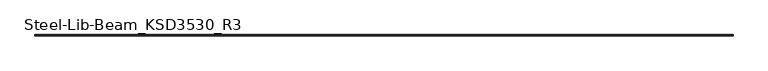
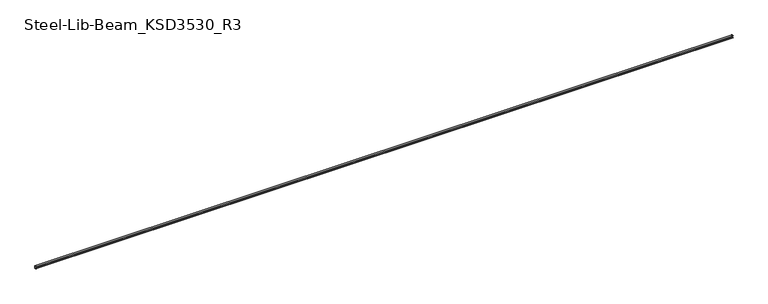
"""IFC4 building model written with IfcOpenShell, lengths in millimetres: beam geometry, Steel-Lib-Beam_KSD3530_R3 : BMS291_C-150×75x20x4.5."""

from ifc_helpers import new_model, si_unit, point, frame, frame_2d, origin, place, context, project, spatial, polyline, circle_curve, trimmed, segment, composite_curve, outline, extrude, source, transform, mapped, element, save


def steel_lib_beam_ksd3530_r3_05cad94e(model_context):
    return source(origin(), model_context, "Body", "SweptSolid", [
        extrude(outline(composite_curve([segment(trimmed(circle_curve(frame_2d((-41.0, 66.0)), 9.0), [point((-50.0, 66.0))], [point((-41.0, 75.0))], False, "CARTESIAN"), True, "CONTINUOUS"), segment(polyline([(-41.0, 75.0), (16.0, 75.0)]), True, "CONTINUOUS"), segment(trimmed(circle_curve(frame_2d((16.0, 66.0)), 9.0), [point((16.0, 75.0))], [point((25.0, 66.0))], False, "CARTESIAN"), True, "CONTINUOUS"), segment(polyline([(25.0, 66.0), (25.0, -66.0)]), True, "CONTINUOUS"), segment(trimmed(circle_curve(frame_2d((16.0, -66.0)), 9.0), [point((25.0, -66.0))], [point((16.0, -75.0))], False, "CARTESIAN"), True, "CONTINUOUS"), segment(polyline([(16.0, -75.0), (-41.0, -75.0)]), True, "CONTINUOUS"), segment(trimmed(circle_curve(frame_2d((-41.0, -66.0)), 9.0), [point((-41.0, -75.0))], [point((-50.0, -66.0))], False, "CARTESIAN"), True, "CONTINUOUS"), segment(polyline([(-50.0, -66.0), (-50.0, -55.0), (-45.5, -55.0), (-45.5, -66.0)]), True, "CONTINUOUS"), segment(trimmed(circle_curve(frame_2d((-41.0, -66.0)), 4.5), [point((-45.5, -66.0))], [point((-41.0, -70.5))], True, "CARTESIAN"), True, "CONTINUOUS"), segment(polyline([(-41.0, -70.5), (16.0, -70.5)]), True, "CONTINUOUS"), segment(trimmed(circle_curve(frame_2d((16.0, -66.0)), 4.5), [point((16.0, -70.5))], [point((20.5, -66.0))], True, "CARTESIAN"), True, "CONTINUOUS"), segment(polyline([(20.5, -66.0), (20.5, 66.0)]), True, "CONTINUOUS"), segment(trimmed(circle_curve(frame_2d((16.0, 66.0)), 4.5), [point((20.5, 66.0))], [point((16.0, 70.5))], True, "CARTESIAN"), True, "CONTINUOUS"), segment(polyline([(16.0, 70.5), (-41.0, 70.5)]), True, "CONTINUOUS"), segment(trimmed(circle_curve(frame_2d((-41.0, 66.0)), 4.5), [point((-41.0, 70.5))], [point((-45.5, 66.0))], True, "CARTESIAN"), True, "CONTINUOUS"), segment(polyline([(-45.5, 66.0), (-45.5, 55.0), (-50.0, 55.0), (-50.0, 66.0)]), True, "CONTINUOUS")], self_intersect=False)), frame((-20622.5, 0.0, 0.0), z_axis=(1.0, 0.0, 0.0), x_axis=(0.0, 1.0, 0.0)), (0.0, 0.0, 1.0), 41245.0),
    ])


if __name__ == "__main__":
    model = new_model("IFC4")
    model_context = context("Model", 3, world=origin())
    ifc_project = project(units=[si_unit("LENGTHUNIT", "METRE", prefix="MILLI")], contexts=[model_context])
    site = spatial("IfcSite", under=ifc_project)
    building = spatial("IfcBuilding", under=site)
    placement = place(None, origin())
    steel_lib_beam_ksd3530_r3_shape = steel_lib_beam_ksd3530_r3_05cad94e(model_context)
    element("IfcBeam", 1, ObjectType="Steel-Lib-Beam_KSD3530_R3 : BMS291_C-150×75x20x4.5", at=placement, inside=building, context=model_context, shape_type="MappedRepresentation", body=[
        mapped(steel_lib_beam_ksd3530_r3_shape, transform((0.0, 0.0, 0.0), x_axis=(1.0, 0.0, 0.0), y_axis=(0.0, 1.0, 0.0), z_axis=(0.0, 0.0, 1.0))),
    ])
    save(model, "model.ifc")

# Revit data of these elements
# Type "Steel-Lib-Beam_KSD3530_R3 : BMS291_C-150×75x20x4.5"
#   Keynote = "C-150×75x20x4.5"
#   SteelWeight = "Light"
#   x = 0.0250 m
#   t1 = 0.0090 m
#   t = 0.0045 m
#   Surface Area = 0.629834 m²/m
#   Section Area = 13.9688 cm²
#   Mass per Unit Length = 10.9655 kg/m
#   C = 0.0200 m
#   A = 0.0750 m
#   Length [instance default] = 1.5000 m
#   H = 0.1500 m
#   hec_material4 [instance default] = none
#   hec_material3 [instance default] = none
#   hec_material2 [instance default] = none
#   hec_material1 [instance default] = none
#   Structural Material [instance default] = Metal - Steel - Light Gauge
#   Assembly Code = ""
# Element 1 (IfcBeam, "Steel-Lib-Beam_KSD3530_R3 : BMS291_C-150×75x20x4.5")
#   Structural Material = none
# Materials
#   "Metal - Steel - Light Gauge": class "Metal", colour RGB 247 247 247, transparency 0
